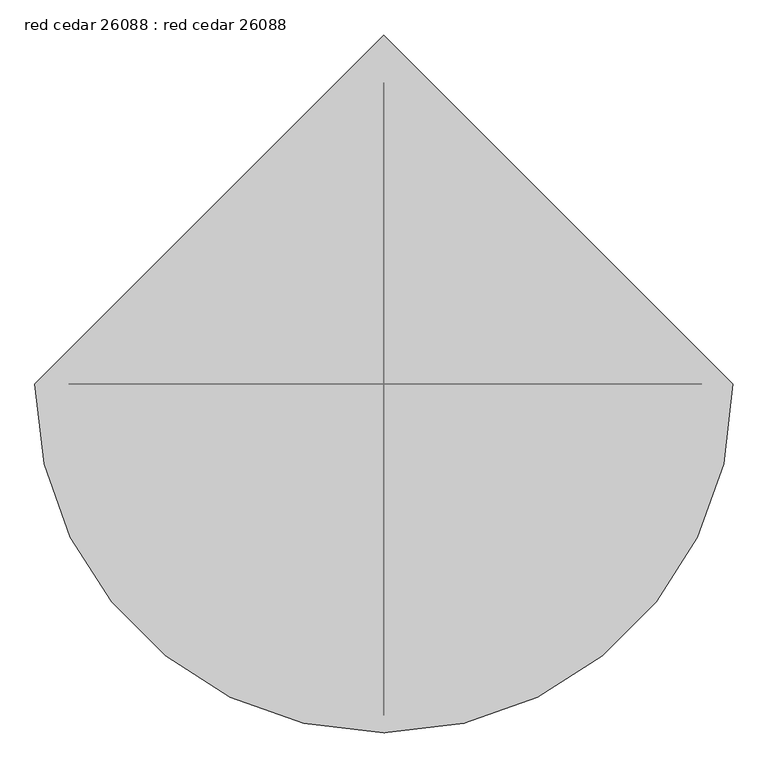
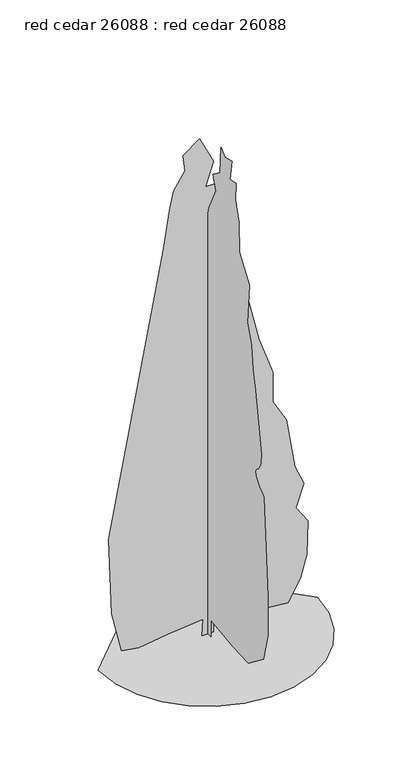
"""IFC4 building model written with IfcOpenShell, lengths in millimetres: proxy geometry, red cedar 26088 : red cedar 26088."""

import ifcopenshell
import ifcopenshell.guid

model = None  # the IFC model being written
_history = None  # IfcOwnerHistory: only IFC2X3 demands one
_inside = {}  # id of a spatial element -> (the spatial element, [elements in it])
_under = {}  # id of a project, library or spatial element -> (it, [spatial elements below it])
_declared = {}  # id of a project -> (the project, [libraries it declares])
_typed = {}  # id of a type object -> (the type object, [elements of that type])
_made_of = {}  # id of a material, layer set ... -> (it, [elements and type objects made of it])


def new_model(schema):
    """Start an empty IFC model of exactly this schema.

    Asked for "IFC4X3", IfcOpenShell would pick the latest addendum, in which some entities
    have other attributes; the version numbers below select the first issue.
    IFC2X3 requires an IfcOwnerHistory on every rooted entity: one is made here for all.
    """
    global model, _history
    if schema == "IFC4X3":
        model = ifcopenshell.file(schema_version=(4, 3, 0, 0))
    else:
        model = ifcopenshell.file(schema=schema)
    _inside.clear()
    _under.clear()
    _declared.clear()
    _typed.clear()
    _made_of.clear()
    _history = None
    if model.schema == "IFC2X3":
        org = make("IfcOrganization", Name="unknown")
        user = make(
            "IfcPersonAndOrganization",
            ThePerson=make("IfcPerson", FamilyName="unknown"),
            TheOrganization=org,
        )
        app = make(
            "IfcApplication",
            ApplicationDeveloper=org,
            Version="unknown",
            ApplicationFullName="unknown",
            ApplicationIdentifier="unknown",
        )
        _history = make(
            "IfcOwnerHistory",
            OwningUser=user,
            OwningApplication=app,
            ChangeAction="ADDED",
            CreationDate=0,
        )
    return model


def make(cls, **values):
    """One entity of the class cls with the attributes given. An attribute that is None is left unset."""
    return model.create_entity(
        cls, **{name: value for name, value in values.items() if value is not None}
    )


def rooted(cls, **values):
    """An entity with a GlobalId (a new one), such as an element, a storey or a relation."""
    return make(cls, GlobalId=ifcopenshell.guid.new(), OwnerHistory=_history, **values)


def si_unit(unit_type, name, prefix=None):
    """IfcSIUnit, for example si_unit("LENGTHUNIT", "METRE", prefix="MILLI")."""
    return make("IfcSIUnit", UnitType=unit_type, Prefix=prefix, Name=name)


def assignment(units):
    """IfcUnitAssignment: the units of a project."""
    return None if units is None else make("IfcUnitAssignment", Units=units)


def point(xyz):
    """IfcCartesianPoint."""
    return None if xyz is None else make("IfcCartesianPoint", Coordinates=xyz)


def direction(xyz):
    """IfcDirection."""
    return None if xyz is None else make("IfcDirection", DirectionRatios=xyz)


def frame(location, z_axis=None, x_axis=None):
    """IfcAxis2Placement3D, a coordinate frame: its origin and axes. An axis left out is left unset."""
    return make(
        "IfcAxis2Placement3D",
        Location=point(location),
        Axis=direction(z_axis),
        RefDirection=direction(x_axis),
    )


def origin():
    """The frame at (0, 0, 0) with its axes left unset."""
    return frame((0.0, 0.0, 0.0))


def place(relative_to, where):
    """IfcLocalPlacement: puts the frame where relative to a parent placement (None: the world)."""
    return make(
        "IfcLocalPlacement", PlacementRelTo=relative_to, RelativePlacement=where
    )


def context(
    kind, dimensions, precision=None, world=None, true_north=None, identifier=None
):
    """IfcGeometricRepresentationContext, for example the 3D "Model" context."""
    return make(
        "IfcGeometricRepresentationContext",
        ContextIdentifier=identifier,
        ContextType=kind,
        CoordinateSpaceDimension=dimensions,
        Precision=precision,
        WorldCoordinateSystem=world,
        TrueNorth=true_north,
    )


def project(units=None, contexts=None):
    """IfcProject with its units and contexts."""
    return rooted(
        "IfcProject",
        Name="project",
        RepresentationContexts=contexts,
        UnitsInContext=assignment(units),
    )


def spatial(cls, under=None, at=None, **own):
    """A site, building, storey or space (cls), placed at a placement, below another one or the project."""
    s = rooted(cls, ObjectPlacement=at, **own)
    if under is not None:
        _under.setdefault(under.id(), (under, []))[1].append(s)
    return s


def point_list(points):
    """IfcCartesianPointList2D or 3D."""
    cls = (
        "IfcCartesianPointList2D" if len(points[0]) == 2 else "IfcCartesianPointList3D"
    )
    return make(cls, CoordList=points)


def triangles(points, corners, closed=None, point_numbers=None):
    """IfcTriangulatedFaceSet: each triangle names its three corners, points numbered from 1."""
    return make(
        "IfcTriangulatedFaceSet",
        Coordinates=point_list(points),
        Closed=closed,
        CoordIndex=corners,
        PnIndex=point_numbers,
    )


def shape(context_of_items, identifier, shape_type, items):
    """IfcShapeRepresentation: the items that make up one representation, for example the "Body"."""
    return make(
        "IfcShapeRepresentation",
        ContextOfItems=context_of_items,
        RepresentationIdentifier=identifier,
        RepresentationType=shape_type,
        Items=items,
    )


def source(mapping_origin, context_of_items, identifier, shape_type, items):
    """IfcRepresentationMap: a shape defined once, which mapped items show again and again."""
    return make(
        "IfcRepresentationMap",
        MappingOrigin=mapping_origin,
        MappedRepresentation=shape(context_of_items, identifier, shape_type, items),
    )


def transform(
    local_origin,
    x_axis=None,
    y_axis=None,
    z_axis=None,
    scale=None,
    scale2=None,
    scale3=None,
    uniform=True,
):
    """IfcCartesianTransformationOperator3D, or its non-uniform kind. x_axis, y_axis, z_axis: its Axis1, 2, 3."""
    if uniform:
        return make(
            "IfcCartesianTransformationOperator3D",
            Axis1=direction(x_axis),
            Axis2=direction(y_axis),
            LocalOrigin=point(local_origin),
            Scale=scale,
            Axis3=direction(z_axis),
        )
    return make(
        "IfcCartesianTransformationOperator3DnonUniform",
        Axis1=direction(x_axis),
        Axis2=direction(y_axis),
        LocalOrigin=point(local_origin),
        Scale=scale,
        Axis3=direction(z_axis),
        Scale2=scale2,
        Scale3=scale3,
    )


def mapped(mapping_source, mapping_target):
    """IfcMappedItem: shows the shape of a source again, moved by a transform."""
    return make(
        "IfcMappedItem", MappingSource=mapping_source, MappingTarget=mapping_target
    )


def made_of(thing, what):
    """Note that an element or type object is made of a material, layer set ...; save() writes the relation."""
    if what is not None:
        _made_of.setdefault(what.id(), (what, []))[1].append(thing)
    return thing


def element(
    cls,
    number,
    at=None,
    inside=None,
    cuts=None,
    type_object=None,
    material=None,
    context=None,
    identifier="Body",
    shape_type=None,
    held_by="IfcProductDefinitionShape",
    body=None,
    shapes=None,
    **own,
):
    """One element of the class cls, such as IfcWall. Its Tag is "e" and its number.

    at: its placement. inside: the storey or other place that contains it. cuts: it is an
    opening in that element (IfcRelVoidsElement). A single representation is given by context,
    identifier, shape_type and body (its items); several are given by shapes. held_by: the class
    of the entity that holds the representations. save() writes the other relations.
    """
    e = rooted(cls, Tag="e%d" % number, ObjectPlacement=at, **own)
    if body is not None:
        shapes = [shape(context, identifier, shape_type, body)]
    if shapes is not None:
        e.Representation = make(held_by, Representations=shapes)
    if inside is not None:
        _inside.setdefault(inside.id(), (inside, []))[1].append(e)
    if cuts is not None:
        rooted(
            "IfcRelVoidsElement", RelatingBuildingElement=cuts, RelatedOpeningElement=e
        )
    if type_object is not None:
        _typed.setdefault(type_object.id(), (type_object, []))[1].append(e)
    return made_of(e, material)


def aggregate(whole, parts):
    """IfcRelAggregates: a whole, such as a stair, and the parts it consists of."""
    return rooted("IfcRelAggregates", RelatingObject=whole, RelatedObjects=parts)


def save(model, path):
    """Write the relations noted so far, then the file.

    IfcRelAggregates (storeys below a building ...), IfcRelContainedInSpatialStructure (elements
    in a storey), IfcRelDefinesByType, IfcRelAssociatesMaterial and IfcRelDeclares: one each for
    every whole, place, type object, material and project.
    """
    for whole, parts in _under.values():
        aggregate(whole, parts)
    for where, things in _inside.values():
        rooted(
            "IfcRelContainedInSpatialStructure",
            RelatedElements=things,
            RelatingStructure=where,
        )
    for kind, things in _typed.values():
        rooted("IfcRelDefinesByType", RelatedObjects=things, RelatingType=kind)
    for what, things in _made_of.values():
        rooted("IfcRelAssociatesMaterial", RelatedObjects=things, RelatingMaterial=what)
    for by, libraries in _declared.values():
        rooted("IfcRelDeclares", RelatingContext=by, RelatedDefinitions=libraries)
    model.write(path)


def red_cedar_26088_red_cedar_26088_a2d53891(model_context):
    return source(origin(), model_context, "Body", "Tessellation", [
        triangles([(-33.5074115, 1.5e-06, 2.9e-06), (-28.3324185, -4.6e-06, 98.3225959), (-233.7142045, 5.5e-06, 79.3805562), (-399.8618937, 1.42e-05, 54.911224), (-499.2444177, 1.75e-05, 72.4481351), (-556.1683414, 5.5e-06, 315.6659792), (-571.6927935, -2.13e-05, 776.2313261), (-483.7199292, -5.29e-05, 1241.968087), (-256.0268143, -0.0001341, 2437.3627087), (-219.8026264, -0.0001489, 2659.8870621), (-199.1031631, -0.0001563, 2768.5481621), (-131.829753, -0.0001654, 2872.0531815), (-142.1794938, -0.0001705, 2965.1948799), (-49.0318863, -0.0001789, 3037.6610962), (33.7659849, -0.0001727, 2872.0531815), (-12.8077666, -0.0001623, 2732.3276985), (49.2907141, -0.000165, 2732.3276985), (295.6025418, -0.0001139, 1694.3850941), (375.3077239, -0.0001037, 1464.4872082), (375.3077239, -9.29e-05, 1283.3674496), (452.9300935, -8.83e-05, 1148.821229), (504.6800234, -7.23e-05, 843.5031647), (556.4274098, -6.75e-05, 724.4813599), (509.8539808, -5.74e-05, 589.9350666), (577.1283992, -5.42e-05, 486.4377502), (571.9518983, -4.2e-05, 284.6170386), (535.7289639, -3.24e-05, 150.0712722), (463.2805882, -2.18e-05, 25.8744608), (341.9448257, -1.73e-05, 40.1411272), (173.487521, -9.7e-06, 36.2241947), (33.7659849, -6.7e-06, 87.9728642), (33.7659849, -1.5e-06, 0.0), (1.3e-06, 29.3359728, 9.21e-05), (-6e-07, 39.6857044, 72.4483894), (6.3e-06, 118.2140961, 25.2313837), (8.9e-06, 262.2040898, 67.2733964), (9.3e-06, 231.1559123, 108.6723366), (1.77e-05, 422.6253662, 108.6723366), (2.22e-05, 505.4242367, 129.3717999), (2.81e-05, 520.9487251, 248.3938681), (3.32e-05, 546.8236719, 465.7393044), (3.52e-05, 510.5982305, 548.5356314), (4.13e-05, 515.7747313, 683.0819246), (4.36e-05, 479.5492536, 771.0548252), (4.75e-05, 464.0248014, 1003.9244047), (4.84e-05, 396.7529265, 1091.8973053), (5.8e-05, 303.6035432, 1531.7615902), (6.33e-05, 200.1064449, 1883.6530472), (6.59e-05, 127.6585687, 2142.3977188), (6.55e-05, 91.4343717, 2168.2701221), (7e-05, 60.3851723, 2302.8164154), (7.46e-05, -12.0630389, 2608.147197), (7.78e-05, -84.5113568, 2753.0287605), (7.72e-05, -53.4621528, 2835.8327179), (7.65e-05, -120.7355538, 2887.572583), (8.31e-05, -131.0852854, 3047.9988373), (7.97e-05, -172.484221, 3011.7783737), (7.74e-05, -239.7573677, 3027.2977753), (7.29e-05, -224.2328974, 2908.2733543), (7.09e-05, -281.1575659, 2918.6366753), (6.66e-05, -275.9810469, 2815.1316559), (6.56e-05, -312.2065247, 2701.2888954), (5.74e-05, -317.3804821, 2520.1615791), (5.24e-05, -419.0363411, 2380.6522167), (4.28e-05, -395.0028517, 2137.2211452), (3.63e-05, -436.4023232, 2028.5498714), (3.51e-05, -451.9267754, 1888.8270046), (2.89e-05, -477.8017585, 1774.9817734), (1.64e-05, -534.7256822, 1417.9137428), (1.56e-05, -534.5885176, 1400.1872086), (1.49e-05, -533.6385392, 1382.5493317), (1.43e-05, -531.0579191, 1365.0945831), (1.37e-05, -526.0338072, 1347.911475), (1.33e-05, -517.7508462, 1331.0889553), (1.32e-05, -505.3962951, 1314.7187336), (1.32e-05, -488.1522532, 1298.891938), (1.29e-05, -477.659507, 1280.543058), (1.17e-05, -482.7217343, 1258.2012531), (1e-05, -498.2538168, 1234.3506741), (8.1e-06, -519.178339, 1211.4779423), (6.3e-06, -540.4152695, 1192.0621943), (5e-06, -556.8820696, 1178.5925222), (1e-05, -563.4987805, 1173.5481354), (-1.16e-05, -601.9975571, 589.9350666), (-1.65e-05, -601.9975571, 351.891457), (-2.19e-05, -555.4241281, 181.1204671), (-2.03e-05, -405.3533463, 67.2733964), (-1.33e-05, -250.1068449, 72.4481351), (-2.5e-06, -32.7624306, 103.4973345), (-1.4e-06, -32.7624306, 8.84e-05), (-633.4046516, 0.0, 0.000118), (-616.6584354, -145.1342734, 0.0001086), (-568.9699219, -278.4169084, 9.86e-05), (-494.1517053, -396.0290245, 8.83e-05), (-396.0290245, -494.1517053, 7.82e-05), (-278.4169084, -568.9699219, 6.86e-05), (-145.1342734, -616.6584354, 5.99e-05), (2.78e-05, -633.4046516, 5.26e-05), (145.1342734, -616.6584354, 4.72e-05), (278.4169084, -568.9699219, 0.0001331), (396.0290245, -494.1517053, 0.0001324), (494.1542487, -396.0290245, 0.0001339), (568.9699219, -278.4169084, 4.88e-05), (616.6584354, -145.1342734, 5.47e-05), (633.4046516, 5.54e-05, 6.26e-05), (-8.33e-05, 633.4046516, 0.0001281)], [[13, 14, 15], [12, 13, 15], [12, 15, 16], [11, 12, 16], [32, 1, 2], [31, 32, 2], [10, 11, 16], [16, 17, 18], [10, 16, 18], [9, 10, 18], [8, 9, 18], [8, 18, 19], [8, 19, 20], [7, 8, 20], [7, 20, 21], [7, 21, 22], [6, 7, 22], [6, 22, 23], [6, 23, 24], [5, 6, 24], [4, 5, 24], [3, 4, 24], [2, 3, 24], [31, 2, 24], [30, 31, 24], [29, 30, 24], [29, 24, 25], [29, 25, 26], [29, 26, 27], [29, 27, 28], [55, 56, 57], [35, 36, 37], [57, 58, 59], [55, 57, 59], [59, 60, 61], [89, 90, 33], [89, 33, 34], [53, 54, 55], [55, 59, 61], [53, 55, 61], [53, 61, 62], [52, 53, 62], [52, 62, 63], [51, 52, 63], [51, 63, 64], [51, 64, 65], [50, 51, 65], [38, 39, 40], [34, 35, 37], [50, 65, 66], [50, 66, 67], [49, 50, 67], [48, 49, 67], [48, 67, 68], [47, 48, 68], [47, 68, 69], [46, 47, 69], [46, 69, 70], [46, 70, 71], [46, 71, 72], [46, 72, 73], [46, 73, 74], [46, 74, 75], [46, 75, 76], [46, 76, 77], [46, 77, 78], [46, 78, 79], [46, 79, 80], [37, 38, 40], [37, 40, 41], [37, 41, 42], [46, 80, 81], [82, 83, 84], [34, 37, 42], [89, 34, 42], [89, 42, 43], [89, 43, 44], [45, 46, 81], [44, 45, 81], [89, 44, 81], [88, 89, 81], [88, 81, 82], [88, 82, 84], [88, 84, 85], [88, 85, 86], [88, 86, 87], [105, 106, 91], [104, 105, 91], [104, 91, 92], [103, 104, 92], [103, 92, 93], [103, 93, 94], [102, 103, 94], [101, 102, 94], [101, 94, 95], [101, 95, 96], [101, 96, 97], [101, 97, 98], [101, 98, 99], [101, 99, 100]], closed=False),
    ])


if __name__ == "__main__":
    model = new_model("IFC4")
    model_context = context("Model", 3, world=origin())
    ifc_project = project(units=[si_unit("LENGTHUNIT", "METRE", prefix="MILLI")], contexts=[model_context])
    site = spatial("IfcSite", under=ifc_project)
    building = spatial("IfcBuilding", under=site)
    placement = place(None, origin())
    red_cedar_26088_red_cedar_26088_shape = red_cedar_26088_red_cedar_26088_a2d53891(model_context)
    element("IfcBuildingElementProxy", 1, Name="red cedar 26088 : red cedar 26088", ObjectType="red cedar 26088 : red cedar 26088", at=placement, inside=building, context=model_context, shape_type="MappedRepresentation", body=[
        mapped(red_cedar_26088_red_cedar_26088_shape, transform((0.0, 0.0, 0.0), x_axis=(1.0, 0.0, 0.0), y_axis=(0.0, 1.0, 0.0), z_axis=(0.0, 0.0, 1.0))),
    ])
    save(model, "model.ifc")

# Revit data of these elements
# Type "red cedar 26088 : red cedar 26088"
#   built-in parameter 1005195 = "RPC-16-FXGH-CPG0-PPQ3-C000-ST1L-LVER-AU"
#   Height = 0
